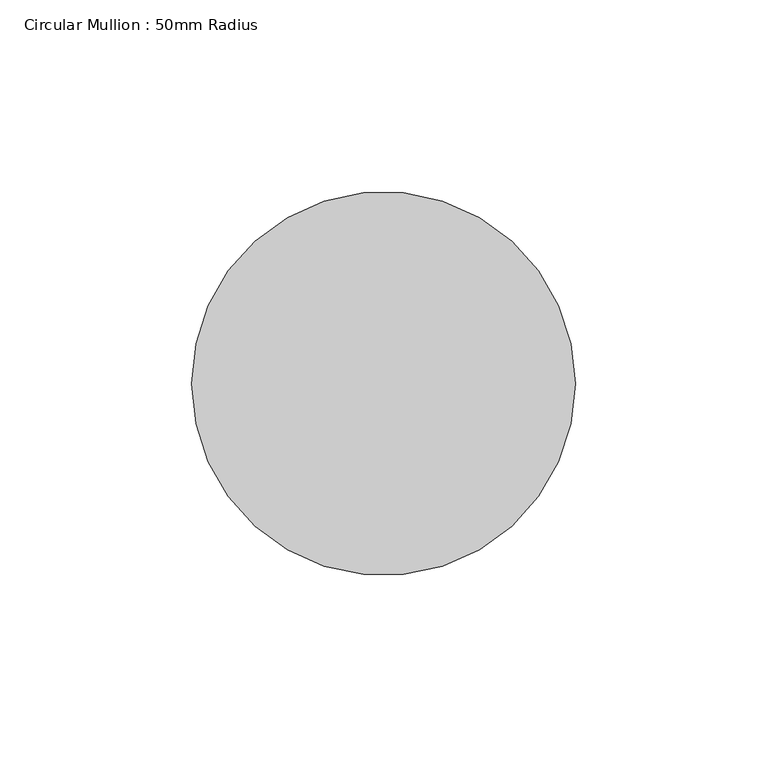
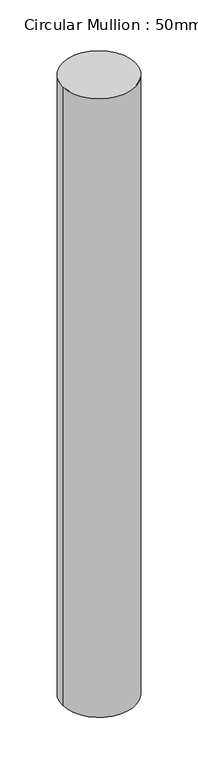
"""IFC4 building model written with IfcOpenShell, lengths in millimetres: member geometry, Circular Mullion : 50mm Radius."""

from ifc_helpers import new_model, si_unit, point, frame, origin, origin_2d, place, context, project, spatial, circle_curve, trimmed, segment, composite_curve, outline, extrude, source, transform, mapped, element, save


def circular_mullion_50mm_radius_3931666a(model_context):
    return source(origin(), model_context, "Body", "SweptSolid", [
        extrude(outline(composite_curve([segment(trimmed(circle_curve(origin_2d(), 50.0), [point((50.0, 0.0))], [point((-50.0, 0.0))], False, "CARTESIAN"), True, "CONTINUOUS"), segment(trimmed(circle_curve(origin_2d(), 50.0), [point((-50.0, 0.0))], [point((50.0, 0.0))], False, "CARTESIAN"), True, "CONTINUOUS")], self_intersect=False)), frame((0.0, 0.0, -903.0835397), z_axis=(0.0, 0.0, 1.0), x_axis=(1.0, 0.0, 0.0)), (0.0, 0.0, 1.0), 903.0835397),
    ])


if __name__ == "__main__":
    model = new_model("IFC4")
    model_context = context("Model", 3, world=origin())
    ifc_project = project(units=[si_unit("LENGTHUNIT", "METRE", prefix="MILLI")], contexts=[model_context])
    site = spatial("IfcSite", under=ifc_project)
    building = spatial("IfcBuilding", under=site)
    placement = place(None, origin())
    circular_mullion_50mm_radius_shape = circular_mullion_50mm_radius_3931666a(model_context)
    element("IfcMember", 1, ObjectType="Circular Mullion : 50mm Radius", at=placement, inside=building, context=model_context, shape_type="MappedRepresentation", body=[
        mapped(circular_mullion_50mm_radius_shape, transform((0.0, 0.0, 0.0), x_axis=(1.0, 0.0, 0.0), y_axis=(0.0, 1.0, 0.0), z_axis=(0.0, 0.0, 1.0))),
    ])
    save(model, "model.ifc")

# Revit data of these elements
# Type "Circular Mullion : 50mm Radius"
#   built-in parameter 1007350 = 0.164042 (stored number, unit not read)
# Element 1 (IfcMember, "Circular Mullion : 50mm Radius")
#   Materials on its faces: "Aluminium"
# Materials
#   "Aluminium": class "Metal", colour RGB 247 247 247, transparency 0, Description = "Aluminium 6061", Cost = 0
